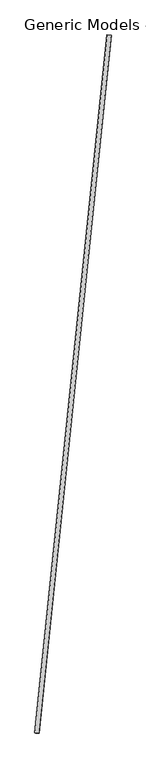
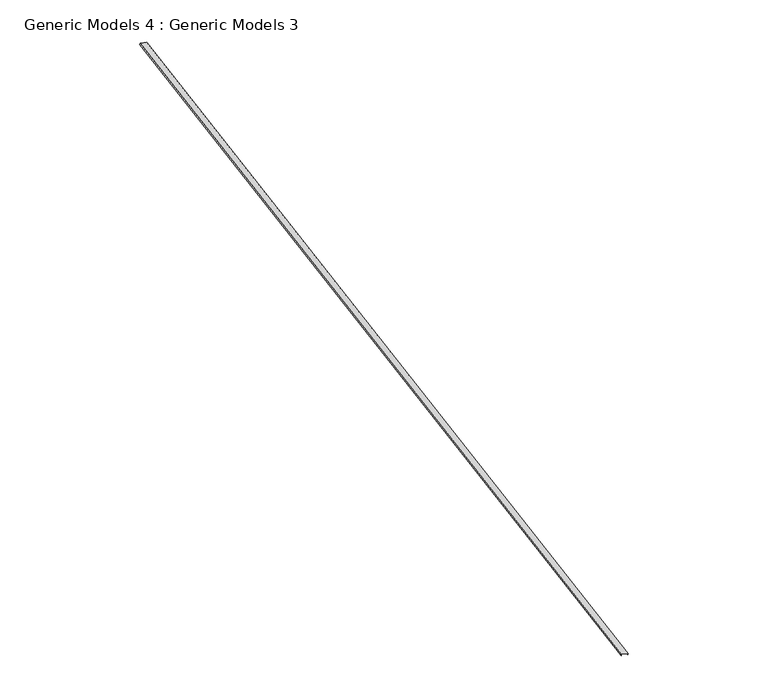
"""IFC4 building model written with IfcOpenShell, lengths in millimetres: proxy geometry, Generic Models 4 : Generic Models 3."""

from ifc_helpers import new_model, si_unit, frame, origin, place, context, project, spatial, polyline, outline, extrude, source, transform, mapped, element, save


def generic_models_4_generic_models_3_e463796e(model_context):
    return source(origin(), model_context, "Body", "SweptSolid", [
        extrude(outline(polyline([(97.4646066, 1e-07), (99.1654809, -17.6103727), (97.5853339, -17.762989), (96.0230459, -1.5874999), (4.088793, -1.5875), (5.8286824, -19.601823), (4.2485354, -19.7544393), (2.3405791, 1e-07), (97.4646066, 1e-07)])), frame((35226.7045536, 40704.3905273, 272198.2577108), z_axis=(-0.10293344407674773, -0.9946674410191907, 0.006433340254794669), x_axis=(0.9820274637778519, -0.10264978490500677, -0.15838270753145897)), (0.0, 0.0, 1.0), 15089.019704),
    ])


if __name__ == "__main__":
    model = new_model("IFC4")
    model_context = context("Model", 3, world=origin())
    ifc_project = project(units=[si_unit("LENGTHUNIT", "METRE", prefix="MILLI")], contexts=[model_context])
    site = spatial("IfcSite", under=ifc_project)
    building = spatial("IfcBuilding", under=site)
    placement = place(None, origin())
    generic_models_4_generic_models_3_shape = generic_models_4_generic_models_3_e463796e(model_context)
    element("IfcBuildingElementProxy", 1, Name="Generic Models 4 : Generic Models 3", ObjectType="Generic Models 4 : Generic Models 3", at=placement, inside=building, context=model_context, shape_type="MappedRepresentation", body=[
        mapped(generic_models_4_generic_models_3_shape, transform((0.0, 0.0, 0.0), x_axis=(1.0, 0.0, 0.0), y_axis=(0.0, 1.0, 0.0), z_axis=(0.0, 0.0, 1.0))),
    ])
    save(model, "model.ifc")

# Revit data of these elements
# Element 1 (IfcBuildingElementProxy, "Generic Models 4 : Generic Models 3")
#   Materials on its faces: "PERFORATED GALV. GUTTER GUARD"
# Materials
#   "PERFORATED GALV. GUTTER GUARD": class "Generic", colour RGB 185 185 185, transparency 0, Cost = 0
